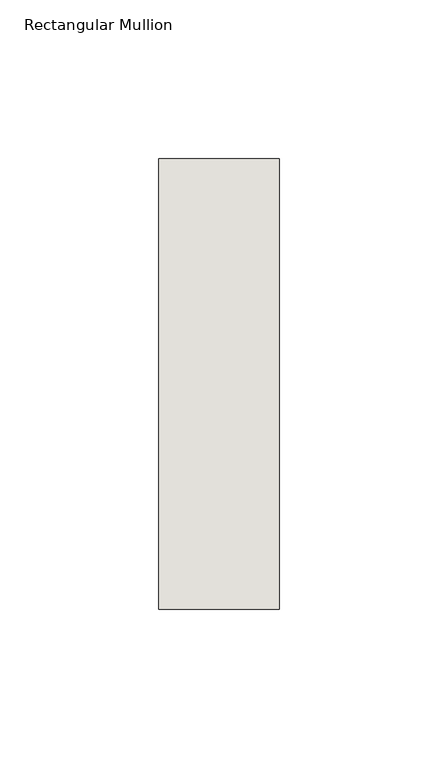
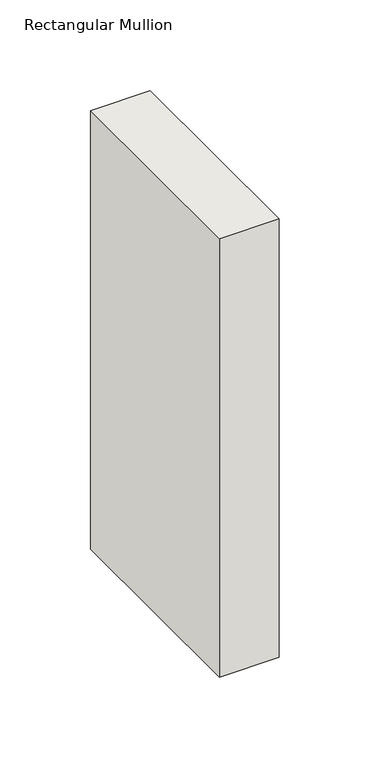
"""IFC4 building model written with IfcOpenShell, lengths in millimetres: wall geometry, Rectangular Mullion : NLRS_21_CWM_hsb-regel 38x142_gen_rsf."""

from ifc_helpers import new_model, si_unit, frame, origin, place, context, project, spatial, polyline, outline, extrude, source, transform, mapped, element, save


def rectangular_mullion_4ed20356(model_context):
    return source(origin(), model_context, "Body", "SweptSolid", [
        extrude(outline(polyline([(0.0, -71.0), (-38.0, -71.0), (-38.0, 71.0), (0.0, 71.0), (0.0, -71.0)])), frame((0.0, 0.0, -295.0), z_axis=(0.0, 0.0, 1.0), x_axis=(1.0, 0.0, 0.0)), (0.0, 0.0, 1.0), 295.0),
    ])


if __name__ == "__main__":
    model = new_model("IFC4")
    model_context = context("Model", 3, world=origin())
    ifc_project = project(units=[si_unit("LENGTHUNIT", "METRE", prefix="MILLI")], contexts=[model_context])
    site = spatial("IfcSite", under=ifc_project)
    building = spatial("IfcBuilding", under=site)
    placement = place(None, origin())
    rectangular_mullion_shape = rectangular_mullion_4ed20356(model_context)
    element("IfcWall", 1, ObjectType="Rectangular Mullion : NLRS_21_CWM_hsb-regel 38x142_gen_rsf", at=placement, inside=building, context=model_context, shape_type="MappedRepresentation", body=[
        mapped(rectangular_mullion_shape, transform((0.0, 0.0, 0.0), x_axis=(1.0, 0.0, 0.0), y_axis=(0.0, 1.0, 0.0), z_axis=(0.0, 0.0, 1.0))),
    ])
    save(model, "model.ifc")

# Revit data of these elements
# Type "Rectangular Mullion : NLRS_21_CWM_hsb-regel 38x142_gen_rsf"
#   Type IfcGUID = "07M7mRoiH1CR8m_RSKIwpF"
#   Assembly Code = "21.10"
#   IfcExportAs = "IfcWall"
#   built-in parameter 1007322 = 0.465879 (stored number, unit not read)
#   built-in parameter 1007321 = 0.062336 (stored number, unit not read)
#   built-in parameter 1007320 = 0.062336 (stored number, unit not read)
# Element 1 (IfcWall, "Rectangular Mullion : NLRS_21_CWM_hsb-regel 38x142_gen_rsf")
#   Materials on its faces: "NLRS_i2_hout naaldhout vuren_gen_rsf"
# Materials
#   "NLRS_i2_hout naaldhout vuren_gen_rsf": class "I - Hout", colour RGB 234 199 147, transparency 0, Keynote = "i2", Manufacturer = "Revit Standards Foundation", URL = "www.revitstandards.org", Description = "hout vuren", Cost = 0
